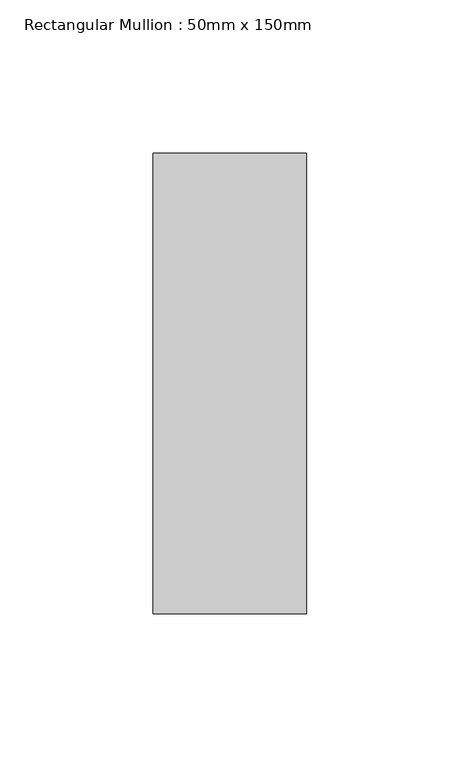
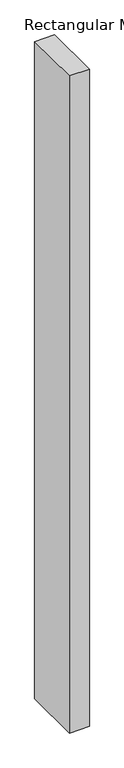
"""IFC4 building model written with IfcOpenShell, lengths in millimetres: member geometry, Rectangular Mullion : 50mm x 150mm."""

from ifc_helpers import new_model, si_unit, frame, origin, place, context, project, spatial, polyline, outline, extrude, source, transform, mapped, element, save


def rectangular_mullion_50mm_x_150mm_86009ec4(model_context):
    return source(origin(), model_context, "Body", "SweptSolid", [
        extrude(outline(polyline([(25.0, 75.0), (25.0, -75.0), (-25.0, -75.0), (-25.0, 75.0), (25.0, 75.0)])), frame((0.0, 0.0, -1736.2355347), z_axis=(0.0, 0.0, 1.0), x_axis=(1.0, 0.0, 0.0)), (0.0, 0.0, 1.0), 1736.2355347),
    ])


if __name__ == "__main__":
    model = new_model("IFC4")
    model_context = context("Model", 3, world=origin())
    ifc_project = project(units=[si_unit("LENGTHUNIT", "METRE", prefix="MILLI")], contexts=[model_context])
    site = spatial("IfcSite", under=ifc_project)
    building = spatial("IfcBuilding", under=site)
    placement = place(None, origin())
    rectangular_mullion_50mm_x_150mm_shape = rectangular_mullion_50mm_x_150mm_86009ec4(model_context)
    element("IfcMember", 1, ObjectType="Rectangular Mullion : 50mm x 150mm", at=placement, inside=building, context=model_context, shape_type="MappedRepresentation", body=[
        mapped(rectangular_mullion_50mm_x_150mm_shape, transform((0.0, 0.0, 0.0), x_axis=(1.0, 0.0, 0.0), y_axis=(0.0, 1.0, 0.0), z_axis=(0.0, 0.0, 1.0))),
    ])
    save(model, "model.ifc")

# Revit data of these elements
# Type "Rectangular Mullion : 50mm x 150mm"
#   built-in parameter 1007304 = 0.492126 (stored number, unit not read)
#   built-in parameter 1007301 = 0.082021 (stored number, unit not read)
#   built-in parameter 1007300 = 0.082021 (stored number, unit not read)
# Element 1 (IfcMember, "Rectangular Mullion : 50mm x 150mm")
#   Materials on its faces: "Aluminum"
# Materials
#   "Aluminum": class "Metal", colour RGB 244 244 244, transparency 0, Description = "Aluminum 6061", Cost = 0
